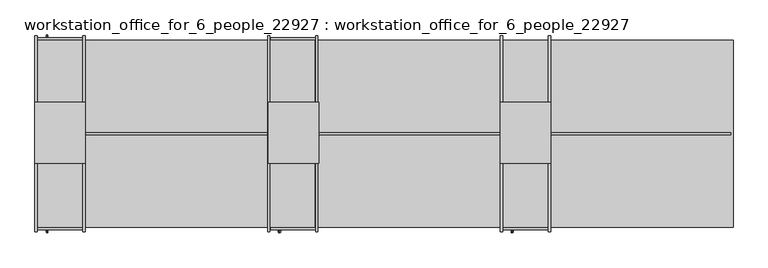
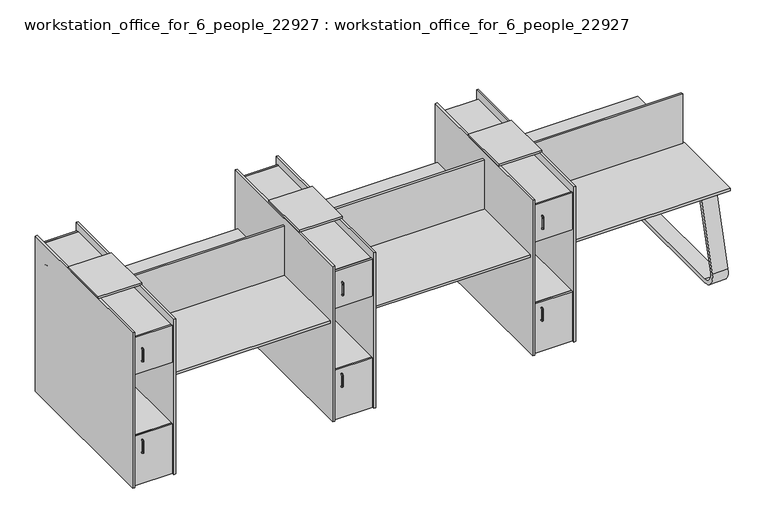
"""IFC4 building model written with IfcOpenShell, lengths in millimetres: proxy geometry, workstation_office_for_6_people_22927 : workstation_office_for_6_people_22927."""

from ifc_helpers import new_model, si_unit, point, frame, frame_2d, origin, origin_with_axes, place, context, project, spatial, polyline, circle_curve, ellipse_curve, trimmed, segment, composite_curve, outline, extrude, source, transform, mapped, element, save
from ifc_brep_helpers import plane_surface, cylinder_surface, revolved_surface, advanced_brep


def workstation_office_for_6_people_22927_workstation_office_for_5136932c(model_context):
    return source(origin(), model_context, "Body", "SolidModel", [
        extrude(outline(polyline([(600.0, 615.0), (600.0, -615.0), (-600.0, -615.0), (-600.0, 615.0), (600.0, 615.0)])), frame((0.0, 0.0, 780.0), z_axis=(0.0, 0.0, 1.0), x_axis=(1.0, 0.0, 0.0)), (0.0, 0.0, 1.0), 20.0),
        extrude(outline(polyline([(2130.0, 615.0), (2130.0, -615.0), (930.0, -615.0), (930.0, 615.0), (2130.0, 615.0)])), frame((0.0, 0.0, 780.0), z_axis=(0.0, 0.0, 1.0), x_axis=(1.0, 0.0, 0.0)), (0.0, 0.0, 1.0), 20.0),
        extrude(outline(polyline([(3660.0, 615.0), (3660.0, -615.0), (2460.0, -615.0), (2460.0, 615.0), (3660.0, 615.0)])), frame((0.0, 0.0, 780.0), z_axis=(0.0, 0.0, 1.0), x_axis=(1.0, 0.0, 0.0)), (0.0, 0.0, 1.0), 20.0),
        extrude(outline(polyline([(600.0, 7.5), (600.0, -7.5), (-600.0, -7.5), (-600.0, 7.5), (600.0, 7.5)])), frame((0.0, 0.0, 400.0), z_axis=(0.0, 0.0, 1.0), x_axis=(1.0, 0.0, 0.0)), (0.0, 0.0, 1.0), 800.0),
        extrude(outline(polyline([(615.0, 645.0), (615.0, -645.0), (600.0, -645.0), (600.0, 645.0), (615.0, 645.0)])), origin_with_axes(), (0.0, 0.0, 1.0), 1256.9637679),
        extrude(outline(polyline([(-615.0, 645.0), (-600.0, 645.0), (-600.0, -645.0), (-615.0, -645.0), (-615.0, 645.0)])), origin_with_axes(), (0.0, 0.0, 1.0), 1256.9637679),
        extrude(outline(polyline([(930.0, 645.0), (930.0, -645.0), (915.0, -645.0), (915.0, 645.0), (930.0, 645.0)])), origin_with_axes(), (0.0, 0.0, 1.0), 1256.9637679),
        extrude(outline(polyline([(-930.0, 645.0), (-915.0, 645.0), (-915.0, -645.0), (-930.0, -645.0), (-930.0, 645.0)])), origin_with_axes(), (0.0, 0.0, 1.0), 1256.9637679),
        extrude(outline(polyline([(2145.0, 645.0), (2145.0, -645.0), (2130.0, -645.0), (2130.0, 645.0), (2145.0, 645.0)])), origin_with_axes(), (0.0, 0.0, 1.0), 1256.9637679),
        extrude(outline(polyline([(2460.0, 645.0), (2460.0, -645.0), (2445.0, -645.0), (2445.0, 645.0), (2460.0, 645.0)])), origin_with_axes(), (0.0, 0.0, 1.0), 1256.9637679),
        extrude(outline(polyline([(-615.0, 615.0), (-615.0, -615.0), (-915.0, -615.0), (-915.0, 615.0), (-615.0, 615.0)])), origin_with_axes(), (0.0, 0.0, 1.0), 400.0),
        extrude(outline(polyline([(615.0, 615.0), (915.0, 615.0), (915.0, -615.0), (615.0, -615.0), (615.0, 615.0)])), origin_with_axes(), (0.0, 0.0, 1.0), 400.0),
        extrude(outline(polyline([(2145.0, 615.0), (2445.0, 615.0), (2445.0, -615.0), (2145.0, -615.0), (2145.0, 615.0)])), origin_with_axes(), (0.0, 0.0, 1.0), 400.0),
        extrude(outline(polyline([(-620.0, 615.0), (-620.0, -615.0), (-920.0, -615.0), (-920.0, 615.0), (-620.0, 615.0)])), frame((0.0, 0.0, 900.0), z_axis=(0.0, 0.0, 1.0), x_axis=(1.0, 0.0, 0.0)), (0.0, 0.0, 1.0), 300.0),
        extrude(outline(polyline([(610.0, 615.0), (910.0, 615.0), (910.0, -615.0), (610.0, -615.0), (610.0, 615.0)])), frame((0.0, 0.0, 900.0), z_axis=(0.0, 0.0, 1.0), x_axis=(1.0, 0.0, 0.0)), (0.0, 0.0, 1.0), 300.0),
        extrude(outline(polyline([(2140.0, 615.0), (2440.0, 615.0), (2440.0, -615.0), (2140.0, -615.0), (2140.0, 615.0)])), frame((0.0, 0.0, 900.0), z_axis=(0.0, 0.0, 1.0), x_axis=(1.0, 0.0, 0.0)), (0.0, 0.0, 1.0), 300.0),
        extrude(outline(polyline([(-620.0, 7.5), (-620.0, -7.5), (-920.0, -7.5), (-920.0, 7.5), (-620.0, 7.5)])), frame((0.0, 0.0, 400.0), z_axis=(0.0, 0.0, 1.0), x_axis=(1.0, 0.0, 0.0)), (0.0, 0.0, 1.0), 500.0),
        extrude(outline(polyline([(610.0, 7.5), (910.0, 7.5), (910.0, -7.5), (610.0, -7.5), (610.0, 7.5)])), frame((0.0, 0.0, 400.0), z_axis=(0.0, 0.0, 1.0), x_axis=(1.0, 0.0, 0.0)), (0.0, 0.0, 1.0), 500.0),
        extrude(outline(polyline([(-620.0, -629.8015658), (-920.0, -629.8015658), (-920.0, -615.0), (-620.0, -615.0), (-620.0, -629.8015658)])), frame((0.0, 0.0, 900.0), z_axis=(0.0, 0.0, 1.0), x_axis=(1.0, 0.0, 0.0)), (0.0, 0.0, 1.0), 300.0),
        extrude(outline(polyline([(-615.0, -629.8015658), (-915.0, -629.8015658), (-915.0, -615.0), (-615.0, -615.0), (-615.0, -629.8015658)])), origin_with_axes(), (0.0, 0.0, 1.0), 400.0),
        extrude(outline(polyline([(920.0, -629.8015658), (620.0, -629.8015658), (620.0, -615.0), (920.0, -615.0), (920.0, -629.8015658)])), frame((0.0, 0.0, 900.0), z_axis=(0.0, 0.0, 1.0), x_axis=(1.0, 0.0, 0.0)), (0.0, 0.0, 1.0), 300.0),
        extrude(outline(polyline([(915.0, -629.8015658), (615.0, -629.8015658), (615.0, -615.0), (915.0, -615.0), (915.0, -629.8015658)])), origin_with_axes(), (0.0, 0.0, 1.0), 400.0),
        extrude(outline(polyline([(2450.0, -629.8015658), (2150.0, -629.8015658), (2150.0, -615.0), (2450.0, -615.0), (2450.0, -629.8015658)])), frame((0.0, 0.0, 900.0), z_axis=(0.0, 0.0, 1.0), x_axis=(1.0, 0.0, 0.0)), (0.0, 0.0, 1.0), 300.0),
        extrude(outline(polyline([(2445.0, -629.8015658), (2145.0, -629.8015658), (2145.0, -615.0), (2445.0, -615.0), (2445.0, -629.8015658)])), origin_with_axes(), (0.0, 0.0, 1.0), 400.0),
        extrude(outline(polyline([(-920.0, 629.8015658), (-620.0, 629.8015658), (-620.0, 615.0), (-920.0, 615.0), (-920.0, 629.8015658)])), frame((0.0, 0.0, 900.0), z_axis=(0.0, 0.0, 1.0), x_axis=(1.0, 0.0, 0.0)), (0.0, 0.0, 1.0), 300.0),
        extrude(outline(polyline([(-915.0, 629.8015658), (-615.0, 629.8015658), (-615.0, 615.0), (-915.0, 615.0), (-915.0, 629.8015658)])), origin_with_axes(), (0.0, 0.0, 1.0), 400.0),
        extrude(outline(polyline([(620.0, 629.8015658), (920.0, 629.8015658), (920.0, 615.0), (620.0, 615.0), (620.0, 629.8015658)])), frame((0.0, 0.0, 900.0), z_axis=(0.0, 0.0, 1.0), x_axis=(1.0, 0.0, 0.0)), (0.0, 0.0, 1.0), 300.0),
        extrude(outline(polyline([(615.0, 629.8015658), (915.0, 629.8015658), (915.0, 615.0), (615.0, 615.0), (615.0, 629.8015658)])), origin_with_axes(), (0.0, 0.0, 1.0), 400.0),
        extrude(outline(polyline([(2130.0, 7.5), (2130.0, -7.5), (930.0, -7.5), (930.0, 7.5), (2130.0, 7.5)])), frame((0.0, 0.0, 400.0), z_axis=(0.0, 0.0, 1.0), x_axis=(1.0, 0.0, 0.0)), (0.0, 0.0, 1.0), 800.0),
        extrude(outline(polyline([(3644.2536992, 7.5), (3644.2536992, -7.5), (2460.0, -7.5), (2460.0, 7.5), (3644.2536992, 7.5)])), frame((0.0, 0.0, 400.0), z_axis=(0.0, 0.0, 1.0), x_axis=(1.0, 0.0, 0.0)), (0.0, 0.0, 1.0), 800.0),
        extrude(outline(composite_curve([segment(polyline([(483.7065392, 0.0), (-483.7065392, 0.0)]), True, "CONTINUOUS"), segment(trimmed(circle_curve(frame_2d((-483.7065392, 100.0)), 100.0), [point((-483.7065392, 0.0))], [point((-580.1112618, 126.5730966))], False, "CARTESIAN"), True, "CONTINUOUS"), segment(polyline([(-580.1112618, 126.5730966), (-420.239467, 706.5730966)]), True, "CONTINUOUS"), segment(trimmed(circle_curve(frame_2d((-323.8347444, 680.0)), 100.0), [point((-420.239467, 706.5730966))], [point((-323.8347444, 780.0))], False, "CARTESIAN"), True, "CONTINUOUS"), segment(polyline([(-323.8347444, 780.0), (323.8347444, 780.0)]), True, "CONTINUOUS"), segment(trimmed(circle_curve(frame_2d((323.8347444, 680.0)), 100.0), [point((323.8347444, 780.0))], [point((420.239467, 706.5730966))], False, "CARTESIAN"), True, "CONTINUOUS"), segment(polyline([(420.239467, 706.5730966), (580.1112618, 126.5730966)]), True, "CONTINUOUS"), segment(trimmed(circle_curve(frame_2d((483.7065392, 100.0)), 100.0), [point((580.1112618, 126.5730966))], [point((483.7065392, 0.0))], False, "CARTESIAN"), True, "CONTINUOUS")], self_intersect=False), holes=[composite_curve([segment(trimmed(circle_curve(frame_2d((-323.8347444, 680.0)), 70.0), [point((-323.8347444, 750.0))], [point((-391.3180502, 698.6011676))], True, "CARTESIAN"), True, "CONTINUOUS"), segment(polyline([(-391.3180502, 698.6011676), (-551.1898451, 118.6011676)]), True, "CONTINUOUS"), segment(trimmed(circle_curve(frame_2d((-483.7065392, 100.0)), 70.0), [point((-551.1898451, 118.6011676))], [point((-483.7065392, 30.0))], True, "CARTESIAN"), True, "CONTINUOUS"), segment(polyline([(-483.7065392, 30.0), (483.7065392, 30.0)]), True, "CONTINUOUS"), segment(trimmed(circle_curve(frame_2d((483.7065392, 100.0)), 70.0), [point((483.7065392, 30.0))], [point((551.1898451, 118.6011676))], True, "CARTESIAN"), True, "CONTINUOUS"), segment(polyline([(551.1898451, 118.6011676), (391.3180502, 698.6011676)]), True, "CONTINUOUS"), segment(trimmed(circle_curve(frame_2d((323.8347444, 680.0)), 70.0), [point((391.3180502, 698.6011676))], [point((323.8347444, 750.0))], True, "CARTESIAN"), True, "CONTINUOUS"), segment(polyline([(323.8347444, 750.0), (-323.8347444, 750.0)]), True, "CONTINUOUS")], self_intersect=False)]), frame((3540.9206772, 0.0, 0.0), z_axis=(1.0, 0.0, 0.0), x_axis=(0.0, 1.0, 0.0)), (0.0, 0.0, 1.0), 119.0793228),
        extrude(outline(polyline([(-930.0, -192.5), (-930.0, 207.5), (-600.0, 207.5), (-600.0, -192.5), (-930.0, -192.5)])), frame((0.0, 0.0, 1256.9637679), z_axis=(0.0, 0.0, 1.0), x_axis=(1.0, 0.0, 0.0)), (0.0, 0.0, 1.0), 16.6578546),
        extrude(outline(polyline([(605.0, -192.5), (605.0, 207.5), (935.0, 207.5), (935.0, -192.5), (605.0, -192.5)])), frame((0.0, 0.0, 1256.9637679), z_axis=(0.0, 0.0, 1.0), x_axis=(1.0, 0.0, 0.0)), (0.0, 0.0, 1.0), 16.6578546),
        extrude(outline(polyline([(2130.0, -192.5), (2130.0, 207.5), (2460.0, 207.5), (2460.0, -192.5), (2130.0, -192.5)])), frame((0.0, 0.0, 1256.9637679), z_axis=(0.0, 0.0, 1.0), x_axis=(1.0, 0.0, 0.0)), (0.0, 0.0, 1.0), 16.6578546),
        advanced_brep(
        [(-850.0, -629.8015658, 1100.0), (-850.0, -629.8015658, 1090.0), (-850.0, -635.0, 1100.0), (-850.0, -635.0, 1090.0), (-850.0, -640.0, 1085.0), (-850.0, -650.0, 1085.0), (-850.0, -650.0, 1005.0), (-850.0, -640.0, 1005.0), (-850.0, -635.0, 1000.0), (-850.0, -635.0, 990.0), (-850.0, -629.8015658, 990.0), (-850.0, -629.8015658, 1000.0)],
        [
            (0, 1, circle_curve(frame((-850.0, -629.8015658, 1095.0), z_axis=(0.0, 1.0, 0.0), x_axis=(0.0, 0.0, -1.0)), 5.0)),
            (1, 0, circle_curve(frame((-850.0, -629.8015658, 1095.0), z_axis=(0.0, 1.0, 0.0), x_axis=(0.0, 0.0, -1.0)), 5.0)),
            (0, 2),
            (2, 3, circle_curve(frame((-850.0, -635.0, 1095.0), z_axis=(0.0, 1.0, 0.0), x_axis=(0.0, 0.0, -1.0)), 5.0)),
            (3, 1),
            (3, 2, circle_curve(frame((-850.0, -635.0, 1095.0), z_axis=(0.0, 1.0, 0.0), x_axis=(0.0, 0.0, -1.0)), 5.0)),
            (4, 3, circle_curve(frame((-850.0, -635.0, 1085.0), z_axis=(-1.0, 0.0, 0.0), x_axis=(0.0, 0.0, 1.0)), 5.0)),
            (2, 5, circle_curve(frame((-850.0, -635.0, 1085.0), z_axis=(1.0, 0.0, 0.0), x_axis=(0.0, 0.0, 1.0)), 15.0)),
            (5, 4, circle_curve(frame((-850.0, -645.0, 1085.0), z_axis=(0.0, 0.0, 1.0), x_axis=(0.0, 1.0, 0.0)), 5.0)),
            (4, 5, circle_curve(frame((-850.0, -645.0, 1085.0), z_axis=(0.0, 0.0, 1.0), x_axis=(0.0, 1.0, 0.0)), 5.0)),
            (5, 6),
            (6, 7, circle_curve(frame((-850.0, -645.0, 1005.0), z_axis=(0.0, 0.0, 1.0), x_axis=(0.0, 1.0, 0.0)), 5.0)),
            (7, 4),
            (7, 6, circle_curve(frame((-850.0, -645.0, 1005.0), z_axis=(0.0, 0.0, 1.0), x_axis=(0.0, 1.0, 0.0)), 5.0)),
            (8, 7, circle_curve(frame((-850.0, -635.0, 1005.0), z_axis=(-1.0, 0.0, 0.0), x_axis=(0.0, -1.0, 0.0)), 5.0)),
            (6, 9, circle_curve(frame((-850.0, -635.0, 1005.0), z_axis=(1.0, 0.0, 0.0), x_axis=(0.0, -1.0, 0.0)), 15.0)),
            (9, 8, circle_curve(frame((-850.0, -635.0, 995.0), z_axis=(0.0, -1.0, 0.0), x_axis=(0.0, 0.0, 1.0)), 5.0)),
            (8, 9, circle_curve(frame((-850.0, -635.0, 995.0), z_axis=(0.0, -1.0, 0.0), x_axis=(0.0, 0.0, 1.0)), 5.0)),
            (10, 11, circle_curve(frame((-850.0, -629.8015658, 995.0), z_axis=(0.0, 1.0, 0.0), x_axis=(0.0, 0.0, 1.0)), 5.0)),
            (11, 10, circle_curve(frame((-850.0, -629.8015658, 995.0), z_axis=(0.0, 1.0, 0.0), x_axis=(0.0, 0.0, 1.0)), 5.0)),
            (9, 10),
            (11, 8),
        ],
        [
            plane_surface(frame((0.0, -629.8015658, 1095.0), z_axis=(0.0, 1.0, 0.0), x_axis=(1.0, 0.0, 0.0))),
            cylinder_surface(frame((-850.0, -629.8015658, 1095.0), z_axis=(0.0, 1.0, 0.0), x_axis=(0.0, 0.0, -1.0)), 5.0),
            revolved_surface(trimmed(ellipse_curve(frame((-850.0, -635.0, 1095.0), z_axis=(0.0, 1.0, 0.0), x_axis=(0.0, 0.0, -1.0)), 5.0, 5.0), [point((-850.0, -635.0, 1100.0))], [point((-850.0, -635.0, 1090.0))], True, "CARTESIAN"), (0.0, -635.0, 1085.0), (1.0, 0.0, 0.0)),
            revolved_surface(trimmed(ellipse_curve(frame((-850.0, -635.0, 1095.0), z_axis=(0.0, 1.0, 0.0), x_axis=(0.0, 0.0, -1.0)), 5.0, 5.0), [point((-850.0, -635.0, 1090.0))], [point((-850.0, -635.0, 1100.0))], True, "CARTESIAN"), (0.0, -635.0, 1085.0), (1.0, 0.0, 0.0)),
            cylinder_surface(frame((-850.0, -645.0, 1085.0), z_axis=(0.0, 0.0, 1.0), x_axis=(0.0, 1.0, 0.0)), 5.0),
            revolved_surface(trimmed(ellipse_curve(frame((-850.0, -645.0, 1005.0), z_axis=(0.0, 0.0, 1.0), x_axis=(0.0, 1.0, 0.0)), 5.0, 5.0), [point((-850.0, -650.0, 1005.0))], [point((-850.0, -640.0, 1005.0))], True, "CARTESIAN"), (0.0, -635.0, 1005.0), (1.0, 0.0, 0.0)),
            revolved_surface(trimmed(ellipse_curve(frame((-850.0, -645.0, 1005.0), z_axis=(0.0, 0.0, 1.0), x_axis=(0.0, 1.0, 0.0)), 5.0, 5.0), [point((-850.0, -640.0, 1005.0))], [point((-850.0, -650.0, 1005.0))], True, "CARTESIAN"), (0.0, -635.0, 1005.0), (1.0, 0.0, 0.0)),
            plane_surface(frame((0.0, -629.8015658, 995.0), z_axis=(0.0, 1.0, 0.0), x_axis=(1.0, 0.0, 0.0))),
            cylinder_surface(frame((-850.0, -635.0, 995.0), z_axis=(0.0, -1.0, 0.0), x_axis=(0.0, 0.0, 1.0)), 5.0),
        ],
        [
            (0, [[1, 2]]),
            (1, [[-1, 3, 4, 5]]),
            (1, [[-2, -5, 6, -3]]),
            (2, [[7, -4, 8, 9]]),
            (3, [[-8, -6, -7, 10]]),
            (4, [[-9, 11, 12, 13]]),
            (4, [[-10, -13, 14, -11]]),
            (5, [[15, -12, 16, 17]]),
            (6, [[-16, -14, -15, 18]]),
            (7, [[19, 20]]),
            (8, [[-17, 21, -20, 22]]),
            (8, [[-18, -22, -19, -21]]),
        ],
    ),
        advanced_brep(
        [(-850.0, -629.8015658, 360.0), (-850.0, -629.8015658, 350.0), (-850.0, -635.0, 360.0), (-850.0, -635.0, 350.0), (-850.0, -640.0, 345.0), (-850.0, -650.0, 345.0), (-850.0, -650.0, 265.0), (-850.0, -640.0, 265.0), (-850.0, -635.0, 260.0), (-850.0, -635.0, 250.0), (-850.0, -629.8015658, 250.0), (-850.0, -629.8015658, 260.0)],
        [
            (0, 1, circle_curve(frame((-850.0, -629.8015658, 355.0), z_axis=(0.0, 1.0, 0.0), x_axis=(0.0, 0.0, -1.0)), 5.0)),
            (1, 0, circle_curve(frame((-850.0, -629.8015658, 355.0), z_axis=(0.0, 1.0, 0.0), x_axis=(0.0, 0.0, -1.0)), 5.0)),
            (0, 2),
            (2, 3, circle_curve(frame((-850.0, -635.0, 355.0), z_axis=(0.0, 1.0, 0.0), x_axis=(0.0, 0.0, -1.0)), 5.0)),
            (3, 1),
            (3, 2, circle_curve(frame((-850.0, -635.0, 355.0), z_axis=(0.0, 1.0, 0.0), x_axis=(0.0, 0.0, -1.0)), 5.0)),
            (4, 3, circle_curve(frame((-850.0, -635.0, 345.0), z_axis=(-1.0, 0.0, 0.0), x_axis=(0.0, 0.0, 1.0)), 5.0)),
            (2, 5, circle_curve(frame((-850.0, -635.0, 345.0), z_axis=(1.0, 0.0, 0.0), x_axis=(0.0, 0.0, 1.0)), 15.0)),
            (5, 4, circle_curve(frame((-850.0, -645.0, 345.0), z_axis=(0.0, 0.0, 1.0), x_axis=(0.0, 1.0, 0.0)), 5.0)),
            (4, 5, circle_curve(frame((-850.0, -645.0, 345.0), z_axis=(0.0, 0.0, 1.0), x_axis=(0.0, 1.0, 0.0)), 5.0)),
            (5, 6),
            (6, 7, circle_curve(frame((-850.0, -645.0, 265.0), z_axis=(0.0, 0.0, 1.0), x_axis=(0.0, 1.0, 0.0)), 5.0)),
            (7, 4),
            (7, 6, circle_curve(frame((-850.0, -645.0, 265.0), z_axis=(0.0, 0.0, 1.0), x_axis=(0.0, 1.0, 0.0)), 5.0)),
            (8, 7, circle_curve(frame((-850.0, -635.0, 265.0), z_axis=(-1.0, 0.0, 0.0), x_axis=(0.0, -1.0, 0.0)), 5.0)),
            (6, 9, circle_curve(frame((-850.0, -635.0, 265.0), z_axis=(1.0, 0.0, 0.0), x_axis=(0.0, -1.0, 0.0)), 15.0)),
            (9, 8, circle_curve(frame((-850.0, -635.0, 255.0), z_axis=(0.0, -1.0, 0.0), x_axis=(0.0, 0.0, 1.0)), 5.0)),
            (8, 9, circle_curve(frame((-850.0, -635.0, 255.0), z_axis=(0.0, -1.0, 0.0), x_axis=(0.0, 0.0, 1.0)), 5.0)),
            (10, 11, circle_curve(frame((-850.0, -629.8015658, 255.0), z_axis=(0.0, 1.0, 0.0), x_axis=(0.0, 0.0, 1.0)), 5.0)),
            (11, 10, circle_curve(frame((-850.0, -629.8015658, 255.0), z_axis=(0.0, 1.0, 0.0), x_axis=(0.0, 0.0, 1.0)), 5.0)),
            (9, 10),
            (11, 8),
        ],
        [
            plane_surface(frame((0.0, -629.8015658, 355.0), z_axis=(0.0, 1.0, 0.0), x_axis=(1.0, 0.0, 0.0))),
            cylinder_surface(frame((-850.0, -629.8015658, 355.0), z_axis=(0.0, 1.0, 0.0), x_axis=(0.0, 0.0, -1.0)), 5.0),
            revolved_surface(trimmed(ellipse_curve(frame((-850.0, -635.0, 355.0), z_axis=(0.0, 1.0, 0.0), x_axis=(0.0, 0.0, -1.0)), 5.0, 5.0), [point((-850.0, -635.0, 360.0))], [point((-850.0, -635.0, 350.0))], True, "CARTESIAN"), (0.0, -635.0, 345.0), (1.0, 0.0, 0.0)),
            revolved_surface(trimmed(ellipse_curve(frame((-850.0, -635.0, 355.0), z_axis=(0.0, 1.0, 0.0), x_axis=(0.0, 0.0, -1.0)), 5.0, 5.0), [point((-850.0, -635.0, 350.0))], [point((-850.0, -635.0, 360.0))], True, "CARTESIAN"), (0.0, -635.0, 345.0), (1.0, 0.0, 0.0)),
            cylinder_surface(frame((-850.0, -645.0, 345.0), z_axis=(0.0, 0.0, 1.0), x_axis=(0.0, 1.0, 0.0)), 5.0),
            revolved_surface(trimmed(ellipse_curve(frame((-850.0, -645.0, 265.0), z_axis=(0.0, 0.0, 1.0), x_axis=(0.0, 1.0, 0.0)), 5.0, 5.0), [point((-850.0, -650.0, 265.0))], [point((-850.0, -640.0, 265.0))], True, "CARTESIAN"), (0.0, -635.0, 265.0), (1.0, 0.0, 0.0)),
            revolved_surface(trimmed(ellipse_curve(frame((-850.0, -645.0, 265.0), z_axis=(0.0, 0.0, 1.0), x_axis=(0.0, 1.0, 0.0)), 5.0, 5.0), [point((-850.0, -640.0, 265.0))], [point((-850.0, -650.0, 265.0))], True, "CARTESIAN"), (0.0, -635.0, 265.0), (1.0, 0.0, 0.0)),
            plane_surface(frame((0.0, -629.8015658, 255.0), z_axis=(0.0, 1.0, 0.0), x_axis=(1.0, 0.0, 0.0))),
            cylinder_surface(frame((-850.0, -635.0, 255.0), z_axis=(0.0, -1.0, 0.0), x_axis=(0.0, 0.0, 1.0)), 5.0),
        ],
        [
            (0, [[1, 2]]),
            (1, [[-1, 3, 4, 5]]),
            (1, [[-2, -5, 6, -3]]),
            (2, [[7, -4, 8, 9]]),
            (3, [[-8, -6, -7, 10]]),
            (4, [[-9, 11, 12, 13]]),
            (4, [[-10, -13, 14, -11]]),
            (5, [[15, -12, 16, 17]]),
            (6, [[-16, -14, -15, 18]]),
            (7, [[19, 20]]),
            (8, [[-17, 21, -20, 22]]),
            (8, [[-18, -22, -19, -21]]),
        ],
    ),
        advanced_brep(
        [(680.0, -629.8015658, 1100.0), (680.0, -629.8015658, 1090.0), (680.0, -635.0, 1100.0), (680.0, -635.0, 1090.0), (680.0, -640.0, 1085.0), (680.0, -650.0, 1085.0), (680.0, -650.0, 1005.0), (680.0, -640.0, 1005.0), (680.0, -635.0, 1000.0), (680.0, -635.0, 990.0), (680.0, -629.8015658, 990.0), (680.0, -629.8015658, 1000.0)],
        [
            (0, 1, circle_curve(frame((680.0, -629.8015658, 1095.0), z_axis=(0.0, 1.0, 0.0), x_axis=(0.0, 0.0, -1.0)), 5.0)),
            (1, 0, circle_curve(frame((680.0, -629.8015658, 1095.0), z_axis=(0.0, 1.0, 0.0), x_axis=(0.0, 0.0, -1.0)), 5.0)),
            (0, 2),
            (2, 3, circle_curve(frame((680.0, -635.0, 1095.0), z_axis=(0.0, 1.0, 0.0), x_axis=(0.0, 0.0, -1.0)), 5.0)),
            (3, 1),
            (3, 2, circle_curve(frame((680.0, -635.0, 1095.0), z_axis=(0.0, 1.0, 0.0), x_axis=(0.0, 0.0, -1.0)), 5.0)),
            (4, 3, circle_curve(frame((680.0, -635.0, 1085.0), z_axis=(-1.0, 0.0, 0.0), x_axis=(0.0, 0.0, 1.0)), 5.0)),
            (2, 5, circle_curve(frame((680.0, -635.0, 1085.0), z_axis=(1.0, 0.0, 0.0), x_axis=(0.0, 0.0, 1.0)), 15.0)),
            (5, 4, circle_curve(frame((680.0, -645.0, 1085.0), z_axis=(0.0, 0.0, 1.0), x_axis=(0.0, 1.0, 0.0)), 5.0)),
            (4, 5, circle_curve(frame((680.0, -645.0, 1085.0), z_axis=(0.0, 0.0, 1.0), x_axis=(0.0, 1.0, 0.0)), 5.0)),
            (5, 6),
            (6, 7, circle_curve(frame((680.0, -645.0, 1005.0), z_axis=(0.0, 0.0, 1.0), x_axis=(0.0, 1.0, 0.0)), 5.0)),
            (7, 4),
            (7, 6, circle_curve(frame((680.0, -645.0, 1005.0), z_axis=(0.0, 0.0, 1.0), x_axis=(0.0, 1.0, 0.0)), 5.0)),
            (8, 7, circle_curve(frame((680.0, -635.0, 1005.0), z_axis=(-1.0, 0.0, 0.0), x_axis=(0.0, -1.0, 0.0)), 5.0)),
            (6, 9, circle_curve(frame((680.0, -635.0, 1005.0), z_axis=(1.0, 0.0, 0.0), x_axis=(0.0, -1.0, 0.0)), 15.0)),
            (9, 8, circle_curve(frame((680.0, -635.0, 995.0), z_axis=(0.0, -1.0, 0.0), x_axis=(0.0, 0.0, 1.0)), 5.0)),
            (8, 9, circle_curve(frame((680.0, -635.0, 995.0), z_axis=(0.0, -1.0, 0.0), x_axis=(0.0, 0.0, 1.0)), 5.0)),
            (10, 11, circle_curve(frame((680.0, -629.8015658, 995.0), z_axis=(0.0, 1.0, 0.0), x_axis=(0.0, 0.0, 1.0)), 5.0)),
            (11, 10, circle_curve(frame((680.0, -629.8015658, 995.0), z_axis=(0.0, 1.0, 0.0), x_axis=(0.0, 0.0, 1.0)), 5.0)),
            (9, 10),
            (11, 8),
        ],
        [
            plane_surface(frame((1530.0, -629.8015658, 1095.0), z_axis=(0.0, 1.0, 0.0), x_axis=(1.0, 0.0, 0.0))),
            cylinder_surface(frame((680.0, -629.8015658, 1095.0), z_axis=(0.0, 1.0, 0.0), x_axis=(0.0, 0.0, -1.0)), 5.0),
            revolved_surface(trimmed(ellipse_curve(frame((680.0, -635.0, 1095.0), z_axis=(0.0, 1.0, 0.0), x_axis=(0.0, 0.0, -1.0)), 5.0, 5.0), [point((680.0, -635.0, 1100.0))], [point((680.0, -635.0, 1090.0))], True, "CARTESIAN"), (1530.0, -635.0, 1085.0), (1.0, 0.0, 0.0)),
            revolved_surface(trimmed(ellipse_curve(frame((680.0, -635.0, 1095.0), z_axis=(0.0, 1.0, 0.0), x_axis=(0.0, 0.0, -1.0)), 5.0, 5.0), [point((680.0, -635.0, 1090.0))], [point((680.0, -635.0, 1100.0))], True, "CARTESIAN"), (1530.0, -635.0, 1085.0), (1.0, 0.0, 0.0)),
            cylinder_surface(frame((680.0, -645.0, 1085.0), z_axis=(0.0, 0.0, 1.0), x_axis=(0.0, 1.0, 0.0)), 5.0),
            revolved_surface(trimmed(ellipse_curve(frame((680.0, -645.0, 1005.0), z_axis=(0.0, 0.0, 1.0), x_axis=(0.0, 1.0, 0.0)), 5.0, 5.0), [point((680.0, -650.0, 1005.0))], [point((680.0, -640.0, 1005.0))], True, "CARTESIAN"), (1530.0, -635.0, 1005.0), (1.0, 0.0, 0.0)),
            revolved_surface(trimmed(ellipse_curve(frame((680.0, -645.0, 1005.0), z_axis=(0.0, 0.0, 1.0), x_axis=(0.0, 1.0, 0.0)), 5.0, 5.0), [point((680.0, -640.0, 1005.0))], [point((680.0, -650.0, 1005.0))], True, "CARTESIAN"), (1530.0, -635.0, 1005.0), (1.0, 0.0, 0.0)),
            plane_surface(frame((1530.0, -629.8015658, 995.0), z_axis=(0.0, 1.0, 0.0), x_axis=(1.0, 0.0, 0.0))),
            cylinder_surface(frame((680.0, -635.0, 995.0), z_axis=(0.0, -1.0, 0.0), x_axis=(0.0, 0.0, 1.0)), 5.0),
        ],
        [
            (0, [[1, 2]]),
            (1, [[-1, 3, 4, 5]]),
            (1, [[-2, -5, 6, -3]]),
            (2, [[7, -4, 8, 9]]),
            (3, [[-8, -6, -7, 10]]),
            (4, [[-9, 11, 12, 13]]),
            (4, [[-10, -13, 14, -11]]),
            (5, [[15, -12, 16, 17]]),
            (6, [[-16, -14, -15, 18]]),
            (7, [[19, 20]]),
            (8, [[-17, 21, -20, 22]]),
            (8, [[-18, -22, -19, -21]]),
        ],
    ),
        advanced_brep(
        [(675.0, -629.8015658, 360.0), (675.0, -629.8015658, 350.0), (675.0, -635.0, 360.0), (675.0, -635.0, 350.0), (675.0, -640.0, 345.0), (675.0, -650.0, 345.0), (675.0, -650.0, 265.0), (675.0, -640.0, 265.0), (675.0, -635.0, 260.0), (675.0, -635.0, 250.0), (675.0, -629.8015658, 250.0), (675.0, -629.8015658, 260.0)],
        [
            (0, 1, circle_curve(frame((675.0, -629.8015658, 355.0), z_axis=(0.0, 1.0, 0.0), x_axis=(0.0, 0.0, -1.0)), 5.0)),
            (1, 0, circle_curve(frame((675.0, -629.8015658, 355.0), z_axis=(0.0, 1.0, 0.0), x_axis=(0.0, 0.0, -1.0)), 5.0)),
            (0, 2),
            (2, 3, circle_curve(frame((675.0, -635.0, 355.0), z_axis=(0.0, 1.0, 0.0), x_axis=(0.0, 0.0, -1.0)), 5.0)),
            (3, 1),
            (3, 2, circle_curve(frame((675.0, -635.0, 355.0), z_axis=(0.0, 1.0, 0.0), x_axis=(0.0, 0.0, -1.0)), 5.0)),
            (4, 3, circle_curve(frame((675.0, -635.0, 345.0), z_axis=(-1.0, 0.0, 0.0), x_axis=(0.0, 0.0, 1.0)), 5.0)),
            (2, 5, circle_curve(frame((675.0, -635.0, 345.0), z_axis=(1.0, 0.0, 0.0), x_axis=(0.0, 0.0, 1.0)), 15.0)),
            (5, 4, circle_curve(frame((675.0, -645.0, 345.0), z_axis=(0.0, 0.0, 1.0), x_axis=(0.0, 1.0, 0.0)), 5.0)),
            (4, 5, circle_curve(frame((675.0, -645.0, 345.0), z_axis=(0.0, 0.0, 1.0), x_axis=(0.0, 1.0, 0.0)), 5.0)),
            (5, 6),
            (6, 7, circle_curve(frame((675.0, -645.0, 265.0), z_axis=(0.0, 0.0, 1.0), x_axis=(0.0, 1.0, 0.0)), 5.0)),
            (7, 4),
            (7, 6, circle_curve(frame((675.0, -645.0, 265.0), z_axis=(0.0, 0.0, 1.0), x_axis=(0.0, 1.0, 0.0)), 5.0)),
            (8, 7, circle_curve(frame((675.0, -635.0, 265.0), z_axis=(-1.0, 0.0, 0.0), x_axis=(0.0, -1.0, 0.0)), 5.0)),
            (6, 9, circle_curve(frame((675.0, -635.0, 265.0), z_axis=(1.0, 0.0, 0.0), x_axis=(0.0, -1.0, 0.0)), 15.0)),
            (9, 8, circle_curve(frame((675.0, -635.0, 255.0), z_axis=(0.0, -1.0, 0.0), x_axis=(0.0, 0.0, 1.0)), 5.0)),
            (8, 9, circle_curve(frame((675.0, -635.0, 255.0), z_axis=(0.0, -1.0, 0.0), x_axis=(0.0, 0.0, 1.0)), 5.0)),
            (10, 11, circle_curve(frame((675.0, -629.8015658, 255.0), z_axis=(0.0, 1.0, 0.0), x_axis=(0.0, 0.0, 1.0)), 5.0)),
            (11, 10, circle_curve(frame((675.0, -629.8015658, 255.0), z_axis=(0.0, 1.0, 0.0), x_axis=(0.0, 0.0, 1.0)), 5.0)),
            (9, 10),
            (11, 8),
        ],
        [
            plane_surface(frame((675.0, -629.8015658, 355.0), z_axis=(0.0, 1.0, 0.0), x_axis=(1.0, 0.0, 0.0))),
            cylinder_surface(frame((675.0, -629.8015658, 355.0), z_axis=(0.0, 1.0, 0.0), x_axis=(0.0, 0.0, -1.0)), 5.0),
            revolved_surface(trimmed(ellipse_curve(frame((675.0, -635.0, 355.0), z_axis=(0.0, 1.0, 0.0), x_axis=(0.0, 0.0, -1.0)), 5.0, 5.0), [point((675.0, -635.0, 360.0))], [point((675.0, -635.0, 350.0))], True, "CARTESIAN"), (675.0, -635.0, 345.0), (1.0, 0.0, 0.0)),
            revolved_surface(trimmed(ellipse_curve(frame((675.0, -635.0, 355.0), z_axis=(0.0, 1.0, 0.0), x_axis=(0.0, 0.0, -1.0)), 5.0, 5.0), [point((675.0, -635.0, 350.0))], [point((675.0, -635.0, 360.0))], True, "CARTESIAN"), (675.0, -635.0, 345.0), (1.0, 0.0, 0.0)),
            cylinder_surface(frame((675.0, -645.0, 345.0), z_axis=(0.0, 0.0, 1.0), x_axis=(0.0, 1.0, 0.0)), 5.0),
            revolved_surface(trimmed(ellipse_curve(frame((675.0, -645.0, 265.0), z_axis=(0.0, 0.0, 1.0), x_axis=(0.0, 1.0, 0.0)), 5.0, 5.0), [point((675.0, -650.0, 265.0))], [point((675.0, -640.0, 265.0))], True, "CARTESIAN"), (675.0, -635.0, 265.0), (1.0, 0.0, 0.0)),
            revolved_surface(trimmed(ellipse_curve(frame((675.0, -645.0, 265.0), z_axis=(0.0, 0.0, 1.0), x_axis=(0.0, 1.0, 0.0)), 5.0, 5.0), [point((675.0, -640.0, 265.0))], [point((675.0, -650.0, 265.0))], True, "CARTESIAN"), (675.0, -635.0, 265.0), (1.0, 0.0, 0.0)),
            plane_surface(frame((675.0, -629.8015658, 255.0), z_axis=(0.0, 1.0, 0.0), x_axis=(1.0, 0.0, 0.0))),
            cylinder_surface(frame((675.0, -635.0, 255.0), z_axis=(0.0, -1.0, 0.0), x_axis=(0.0, 0.0, 1.0)), 5.0),
        ],
        [
            (0, [[1, 2]]),
            (1, [[-1, 3, 4, 5]]),
            (1, [[-2, -5, 6, -3]]),
            (2, [[7, -4, 8, 9]]),
            (3, [[-8, -6, -7, 10]]),
            (4, [[-9, 11, 12, 13]]),
            (4, [[-10, -13, 14, -11]]),
            (5, [[15, -12, 16, 17]]),
            (6, [[-16, -14, -15, 18]]),
            (7, [[19, 20]]),
            (8, [[-17, 21, -20, 22]]),
            (8, [[-18, -22, -19, -21]]),
        ],
    ),
        advanced_brep(
        [(2210.0, -629.8015658, 1100.0), (2210.0, -629.8015658, 1090.0), (2210.0, -635.0, 1100.0), (2210.0, -635.0, 1090.0), (2210.0, -640.0, 1085.0), (2210.0, -650.0, 1085.0), (2210.0, -650.0, 1005.0), (2210.0, -640.0, 1005.0), (2210.0, -635.0, 1000.0), (2210.0, -635.0, 990.0), (2210.0, -629.8015658, 990.0), (2210.0, -629.8015658, 1000.0)],
        [
            (0, 1, circle_curve(frame((2210.0, -629.8015658, 1095.0), z_axis=(0.0, 1.0, 0.0), x_axis=(0.0, 0.0, -1.0)), 5.0)),
            (1, 0, circle_curve(frame((2210.0, -629.8015658, 1095.0), z_axis=(0.0, 1.0, 0.0), x_axis=(0.0, 0.0, -1.0)), 5.0)),
            (0, 2),
            (2, 3, circle_curve(frame((2210.0, -635.0, 1095.0), z_axis=(0.0, 1.0, 0.0), x_axis=(0.0, 0.0, -1.0)), 5.0)),
            (3, 1),
            (3, 2, circle_curve(frame((2210.0, -635.0, 1095.0), z_axis=(0.0, 1.0, 0.0), x_axis=(0.0, 0.0, -1.0)), 5.0)),
            (4, 3, circle_curve(frame((2210.0, -635.0, 1085.0), z_axis=(-1.0, 0.0, 0.0), x_axis=(0.0, 0.0, 1.0)), 5.0)),
            (2, 5, circle_curve(frame((2210.0, -635.0, 1085.0), z_axis=(1.0, 0.0, 0.0), x_axis=(0.0, 0.0, 1.0)), 15.0)),
            (5, 4, circle_curve(frame((2210.0, -645.0, 1085.0), z_axis=(0.0, 0.0, 1.0), x_axis=(0.0, 1.0, 0.0)), 5.0)),
            (4, 5, circle_curve(frame((2210.0, -645.0, 1085.0), z_axis=(0.0, 0.0, 1.0), x_axis=(0.0, 1.0, 0.0)), 5.0)),
            (5, 6),
            (6, 7, circle_curve(frame((2210.0, -645.0, 1005.0), z_axis=(0.0, 0.0, 1.0), x_axis=(0.0, 1.0, 0.0)), 5.0)),
            (7, 4),
            (7, 6, circle_curve(frame((2210.0, -645.0, 1005.0), z_axis=(0.0, 0.0, 1.0), x_axis=(0.0, 1.0, 0.0)), 5.0)),
            (8, 7, circle_curve(frame((2210.0, -635.0, 1005.0), z_axis=(-1.0, 0.0, 0.0), x_axis=(0.0, -1.0, 0.0)), 5.0)),
            (6, 9, circle_curve(frame((2210.0, -635.0, 1005.0), z_axis=(1.0, 0.0, 0.0), x_axis=(0.0, -1.0, 0.0)), 15.0)),
            (9, 8, circle_curve(frame((2210.0, -635.0, 995.0), z_axis=(0.0, -1.0, 0.0), x_axis=(0.0, 0.0, 1.0)), 5.0)),
            (8, 9, circle_curve(frame((2210.0, -635.0, 995.0), z_axis=(0.0, -1.0, 0.0), x_axis=(0.0, 0.0, 1.0)), 5.0)),
            (10, 11, circle_curve(frame((2210.0, -629.8015658, 995.0), z_axis=(0.0, 1.0, 0.0), x_axis=(0.0, 0.0, 1.0)), 5.0)),
            (11, 10, circle_curve(frame((2210.0, -629.8015658, 995.0), z_axis=(0.0, 1.0, 0.0), x_axis=(0.0, 0.0, 1.0)), 5.0)),
            (9, 10),
            (11, 8),
        ],
        [
            plane_surface(frame((3060.0, -629.8015658, 1095.0), z_axis=(0.0, 1.0, 0.0), x_axis=(1.0, 0.0, 0.0))),
            cylinder_surface(frame((2210.0, -629.8015658, 1095.0), z_axis=(0.0, 1.0, 0.0), x_axis=(0.0, 0.0, -1.0)), 5.0),
            revolved_surface(trimmed(ellipse_curve(frame((2210.0, -635.0, 1095.0), z_axis=(0.0, 1.0, 0.0), x_axis=(0.0, 0.0, -1.0)), 5.0, 5.0), [point((2210.0, -635.0, 1100.0))], [point((2210.0, -635.0, 1090.0))], True, "CARTESIAN"), (3060.0, -635.0, 1085.0), (1.0, 0.0, 0.0)),
            revolved_surface(trimmed(ellipse_curve(frame((2210.0, -635.0, 1095.0), z_axis=(0.0, 1.0, 0.0), x_axis=(0.0, 0.0, -1.0)), 5.0, 5.0), [point((2210.0, -635.0, 1090.0))], [point((2210.0, -635.0, 1100.0))], True, "CARTESIAN"), (3060.0, -635.0, 1085.0), (1.0, 0.0, 0.0)),
            cylinder_surface(frame((2210.0, -645.0, 1085.0), z_axis=(0.0, 0.0, 1.0), x_axis=(0.0, 1.0, 0.0)), 5.0),
            revolved_surface(trimmed(ellipse_curve(frame((2210.0, -645.0, 1005.0), z_axis=(0.0, 0.0, 1.0), x_axis=(0.0, 1.0, 0.0)), 5.0, 5.0), [point((2210.0, -650.0, 1005.0))], [point((2210.0, -640.0, 1005.0))], True, "CARTESIAN"), (3060.0, -635.0, 1005.0), (1.0, 0.0, 0.0)),
            revolved_surface(trimmed(ellipse_curve(frame((2210.0, -645.0, 1005.0), z_axis=(0.0, 0.0, 1.0), x_axis=(0.0, 1.0, 0.0)), 5.0, 5.0), [point((2210.0, -640.0, 1005.0))], [point((2210.0, -650.0, 1005.0))], True, "CARTESIAN"), (3060.0, -635.0, 1005.0), (1.0, 0.0, 0.0)),
            plane_surface(frame((3060.0, -629.8015658, 995.0), z_axis=(0.0, 1.0, 0.0), x_axis=(1.0, 0.0, 0.0))),
            cylinder_surface(frame((2210.0, -635.0, 995.0), z_axis=(0.0, -1.0, 0.0), x_axis=(0.0, 0.0, 1.0)), 5.0),
        ],
        [
            (0, [[1, 2]]),
            (1, [[-1, 3, 4, 5]]),
            (1, [[-2, -5, 6, -3]]),
            (2, [[7, -4, 8, 9]]),
            (3, [[-8, -6, -7, 10]]),
            (4, [[-9, 11, 12, 13]]),
            (4, [[-10, -13, 14, -11]]),
            (5, [[15, -12, 16, 17]]),
            (6, [[-16, -14, -15, 18]]),
            (7, [[19, 20]]),
            (8, [[-17, 21, -20, 22]]),
            (8, [[-18, -22, -19, -21]]),
        ],
    ),
        advanced_brep(
        [(2205.0, -629.8015658, 360.0), (2205.0, -629.8015658, 350.0), (2205.0, -635.0, 360.0), (2205.0, -635.0, 350.0), (2205.0, -640.0, 345.0), (2205.0, -650.0, 345.0), (2205.0, -650.0, 265.0), (2205.0, -640.0, 265.0), (2205.0, -635.0, 260.0), (2205.0, -635.0, 250.0), (2205.0, -629.8015658, 250.0), (2205.0, -629.8015658, 260.0)],
        [
            (0, 1, circle_curve(frame((2205.0, -629.8015658, 355.0), z_axis=(0.0, 1.0, 0.0), x_axis=(0.0, 0.0, -1.0)), 5.0)),
            (1, 0, circle_curve(frame((2205.0, -629.8015658, 355.0), z_axis=(0.0, 1.0, 0.0), x_axis=(0.0, 0.0, -1.0)), 5.0)),
            (0, 2),
            (2, 3, circle_curve(frame((2205.0, -635.0, 355.0), z_axis=(0.0, 1.0, 0.0), x_axis=(0.0, 0.0, -1.0)), 5.0)),
            (3, 1),
            (3, 2, circle_curve(frame((2205.0, -635.0, 355.0), z_axis=(0.0, 1.0, 0.0), x_axis=(0.0, 0.0, -1.0)), 5.0)),
            (4, 3, circle_curve(frame((2205.0, -635.0, 345.0), z_axis=(-1.0, 0.0, 0.0), x_axis=(0.0, 0.0, 1.0)), 5.0)),
            (2, 5, circle_curve(frame((2205.0, -635.0, 345.0), z_axis=(1.0, 0.0, 0.0), x_axis=(0.0, 0.0, 1.0)), 15.0)),
            (5, 4, circle_curve(frame((2205.0, -645.0, 345.0), z_axis=(0.0, 0.0, 1.0), x_axis=(0.0, 1.0, 0.0)), 5.0)),
            (4, 5, circle_curve(frame((2205.0, -645.0, 345.0), z_axis=(0.0, 0.0, 1.0), x_axis=(0.0, 1.0, 0.0)), 5.0)),
            (5, 6),
            (6, 7, circle_curve(frame((2205.0, -645.0, 265.0), z_axis=(0.0, 0.0, 1.0), x_axis=(0.0, 1.0, 0.0)), 5.0)),
            (7, 4),
            (7, 6, circle_curve(frame((2205.0, -645.0, 265.0), z_axis=(0.0, 0.0, 1.0), x_axis=(0.0, 1.0, 0.0)), 5.0)),
            (8, 7, circle_curve(frame((2205.0, -635.0, 265.0), z_axis=(-1.0, 0.0, 0.0), x_axis=(0.0, -1.0, 0.0)), 5.0)),
            (6, 9, circle_curve(frame((2205.0, -635.0, 265.0), z_axis=(1.0, 0.0, 0.0), x_axis=(0.0, -1.0, 0.0)), 15.0)),
            (9, 8, circle_curve(frame((2205.0, -635.0, 255.0), z_axis=(0.0, -1.0, 0.0), x_axis=(0.0, 0.0, 1.0)), 5.0)),
            (8, 9, circle_curve(frame((2205.0, -635.0, 255.0), z_axis=(0.0, -1.0, 0.0), x_axis=(0.0, 0.0, 1.0)), 5.0)),
            (10, 11, circle_curve(frame((2205.0, -629.8015658, 255.0), z_axis=(0.0, 1.0, 0.0), x_axis=(0.0, 0.0, 1.0)), 5.0)),
            (11, 10, circle_curve(frame((2205.0, -629.8015658, 255.0), z_axis=(0.0, 1.0, 0.0), x_axis=(0.0, 0.0, 1.0)), 5.0)),
            (9, 10),
            (11, 8),
        ],
        [
            plane_surface(frame((2205.0, -629.8015658, 355.0), z_axis=(0.0, 1.0, 0.0), x_axis=(1.0, 0.0, 0.0))),
            cylinder_surface(frame((2205.0, -629.8015658, 355.0), z_axis=(0.0, 1.0, 0.0), x_axis=(0.0, 0.0, -1.0)), 5.0),
            revolved_surface(trimmed(ellipse_curve(frame((2205.0, -635.0, 355.0), z_axis=(0.0, 1.0, 0.0), x_axis=(0.0, 0.0, -1.0)), 5.0, 5.0), [point((2205.0, -635.0, 360.0))], [point((2205.0, -635.0, 350.0))], True, "CARTESIAN"), (2205.0, -635.0, 345.0), (1.0, 0.0, 0.0)),
            revolved_surface(trimmed(ellipse_curve(frame((2205.0, -635.0, 355.0), z_axis=(0.0, 1.0, 0.0), x_axis=(0.0, 0.0, -1.0)), 5.0, 5.0), [point((2205.0, -635.0, 350.0))], [point((2205.0, -635.0, 360.0))], True, "CARTESIAN"), (2205.0, -635.0, 345.0), (1.0, 0.0, 0.0)),
            cylinder_surface(frame((2205.0, -645.0, 345.0), z_axis=(0.0, 0.0, 1.0), x_axis=(0.0, 1.0, 0.0)), 5.0),
            revolved_surface(trimmed(ellipse_curve(frame((2205.0, -645.0, 265.0), z_axis=(0.0, 0.0, 1.0), x_axis=(0.0, 1.0, 0.0)), 5.0, 5.0), [point((2205.0, -650.0, 265.0))], [point((2205.0, -640.0, 265.0))], True, "CARTESIAN"), (2205.0, -635.0, 265.0), (1.0, 0.0, 0.0)),
            revolved_surface(trimmed(ellipse_curve(frame((2205.0, -645.0, 265.0), z_axis=(0.0, 0.0, 1.0), x_axis=(0.0, 1.0, 0.0)), 5.0, 5.0), [point((2205.0, -640.0, 265.0))], [point((2205.0, -650.0, 265.0))], True, "CARTESIAN"), (2205.0, -635.0, 265.0), (1.0, 0.0, 0.0)),
            plane_surface(frame((2205.0, -629.8015658, 255.0), z_axis=(0.0, 1.0, 0.0), x_axis=(1.0, 0.0, 0.0))),
            cylinder_surface(frame((2205.0, -635.0, 255.0), z_axis=(0.0, -1.0, 0.0), x_axis=(0.0, 0.0, 1.0)), 5.0),
        ],
        [
            (0, [[1, 2]]),
            (1, [[-1, 3, 4, 5]]),
            (1, [[-2, -5, 6, -3]]),
            (2, [[7, -4, 8, 9]]),
            (3, [[-8, -6, -7, 10]]),
            (4, [[-9, 11, 12, 13]]),
            (4, [[-10, -13, 14, -11]]),
            (5, [[15, -12, 16, 17]]),
            (6, [[-16, -14, -15, 18]]),
            (7, [[19, 20]]),
            (8, [[-17, 21, -20, 22]]),
            (8, [[-18, -22, -19, -21]]),
        ],
    ),
        advanced_brep(
        [(-850.0, 629.8015658, 1090.0), (-850.0, 629.8015658, 1100.0), (-850.0, 635.0, 1100.0), (-850.0, 635.0, 1090.0), (-850.0, 640.0, 1085.0), (-850.0, 650.0, 1085.0), (-850.0, 650.0, 1005.0), (-850.0, 640.0, 1005.0), (-850.0, 635.0, 1000.0), (-850.0, 635.0, 990.0), (-850.0, 629.8015658, 1000.0), (-850.0, 629.8015658, 990.0)],
        [
            (0, 1, circle_curve(frame((-850.0, 629.8015658, 1095.0), z_axis=(0.0, -1.0, 0.0), x_axis=(0.0, 0.0, 1.0)), 5.0)),
            (1, 0, circle_curve(frame((-850.0, 629.8015658, 1095.0), z_axis=(0.0, -1.0, 0.0), x_axis=(0.0, 0.0, 1.0)), 5.0)),
            (1, 2),
            (2, 3, circle_curve(frame((-850.0, 635.0, 1095.0), z_axis=(0.0, -1.0, 0.0), x_axis=(0.0, 0.0, 1.0)), 5.0)),
            (3, 0),
            (3, 2, circle_curve(frame((-850.0, 635.0, 1095.0), z_axis=(0.0, -1.0, 0.0), x_axis=(0.0, 0.0, 1.0)), 5.0)),
            (4, 3, circle_curve(frame((-850.0, 635.0, 1085.0), z_axis=(1.0, 0.0, 0.0), x_axis=(0.0, 0.0, 1.0)), 5.0)),
            (2, 5, circle_curve(frame((-850.0, 635.0, 1085.0), z_axis=(-1.0, 0.0, 0.0), x_axis=(0.0, 0.0, 1.0)), 15.0)),
            (5, 4, circle_curve(frame((-850.0, 645.0, 1085.0), z_axis=(0.0, 0.0, 1.0), x_axis=(0.0, 1.0, 0.0)), 5.0)),
            (4, 5, circle_curve(frame((-850.0, 645.0, 1085.0), z_axis=(0.0, 0.0, 1.0), x_axis=(0.0, 1.0, 0.0)), 5.0)),
            (5, 6),
            (6, 7, circle_curve(frame((-850.0, 645.0, 1005.0), z_axis=(0.0, 0.0, 1.0), x_axis=(0.0, 1.0, 0.0)), 5.0)),
            (7, 4),
            (7, 6, circle_curve(frame((-850.0, 645.0, 1005.0), z_axis=(0.0, 0.0, 1.0), x_axis=(0.0, 1.0, 0.0)), 5.0)),
            (8, 7, circle_curve(frame((-850.0, 635.0, 1005.0), z_axis=(1.0, 0.0, 0.0), x_axis=(0.0, 1.0, 0.0)), 5.0)),
            (6, 9, circle_curve(frame((-850.0, 635.0, 1005.0), z_axis=(-1.0, 0.0, 0.0), x_axis=(0.0, 1.0, 0.0)), 15.0)),
            (9, 8, circle_curve(frame((-850.0, 635.0, 995.0), z_axis=(0.0, 1.0, 0.0), x_axis=(0.0, 0.0, -1.0)), 5.0)),
            (8, 9, circle_curve(frame((-850.0, 635.0, 995.0), z_axis=(0.0, 1.0, 0.0), x_axis=(0.0, 0.0, -1.0)), 5.0)),
            (10, 11, circle_curve(frame((-850.0, 629.8015658, 995.0), z_axis=(0.0, -1.0, 0.0), x_axis=(0.0, 0.0, -1.0)), 5.0)),
            (11, 10, circle_curve(frame((-850.0, 629.8015658, 995.0), z_axis=(0.0, -1.0, 0.0), x_axis=(0.0, 0.0, -1.0)), 5.0)),
            (9, 11),
            (10, 8),
        ],
        [
            plane_surface(frame((0.0, 629.8015658, 1095.0), z_axis=(0.0, -1.0, 0.0), x_axis=(1.0, 0.0, 0.0))),
            cylinder_surface(frame((-850.0, 629.8015658, 1095.0), z_axis=(0.0, -1.0, 0.0), x_axis=(0.0, 0.0, 1.0)), 5.0),
            revolved_surface(trimmed(ellipse_curve(frame((-850.0, 635.0, 1095.0), z_axis=(0.0, -1.0, 0.0), x_axis=(0.0, 0.0, 1.0)), 5.0, 5.0), [point((-850.0, 635.0, 1100.0))], [point((-850.0, 635.0, 1090.0))], True, "CARTESIAN"), (0.0, 635.0, 1085.0), (-1.0, 0.0, 0.0)),
            revolved_surface(trimmed(ellipse_curve(frame((-850.0, 635.0, 1095.0), z_axis=(0.0, -1.0, 0.0), x_axis=(0.0, 0.0, 1.0)), 5.0, 5.0), [point((-850.0, 635.0, 1090.0))], [point((-850.0, 635.0, 1100.0))], True, "CARTESIAN"), (0.0, 635.0, 1085.0), (-1.0, 0.0, 0.0)),
            cylinder_surface(frame((-850.0, 645.0, 1085.0), z_axis=(0.0, 0.0, 1.0), x_axis=(0.0, 1.0, 0.0)), 5.0),
            revolved_surface(trimmed(ellipse_curve(frame((-850.0, 645.0, 1005.0), z_axis=(0.0, 0.0, 1.0), x_axis=(0.0, 1.0, 0.0)), 5.0, 5.0), [point((-850.0, 650.0, 1005.0))], [point((-850.0, 640.0, 1005.0))], True, "CARTESIAN"), (0.0, 635.0, 1005.0), (-1.0, 0.0, 0.0)),
            revolved_surface(trimmed(ellipse_curve(frame((-850.0, 645.0, 1005.0), z_axis=(0.0, 0.0, 1.0), x_axis=(0.0, 1.0, 0.0)), 5.0, 5.0), [point((-850.0, 640.0, 1005.0))], [point((-850.0, 650.0, 1005.0))], True, "CARTESIAN"), (0.0, 635.0, 1005.0), (-1.0, 0.0, 0.0)),
            plane_surface(frame((0.0, 629.8015658, 995.0), z_axis=(0.0, -1.0, 0.0), x_axis=(1.0, 0.0, 0.0))),
            cylinder_surface(frame((-850.0, 635.0, 995.0), z_axis=(0.0, 1.0, 0.0), x_axis=(0.0, 0.0, -1.0)), 5.0),
        ],
        [
            (0, [[1, 2]]),
            (1, [[-2, 3, 4, 5]]),
            (1, [[-1, -5, 6, -3]]),
            (2, [[7, -4, 8, 9]]),
            (3, [[-8, -6, -7, 10]]),
            (4, [[-9, 11, 12, 13]]),
            (4, [[-10, -13, 14, -11]]),
            (5, [[15, -12, 16, 17]]),
            (6, [[-16, -14, -15, 18]]),
            (7, [[19, 20]]),
            (8, [[-17, 21, -19, 22]]),
            (8, [[-18, -22, -20, -21]]),
        ],
    ),
    ])


if __name__ == "__main__":
    model = new_model("IFC4")
    model_context = context("Model", 3, world=origin())
    ifc_project = project(units=[si_unit("LENGTHUNIT", "METRE", prefix="MILLI")], contexts=[model_context])
    site = spatial("IfcSite", under=ifc_project)
    building = spatial("IfcBuilding", under=site)
    placement = place(None, origin())
    workstation_office_for_6_people_22927_workstation_office_for_shape = workstation_office_for_6_people_22927_workstation_office_for_5136932c(model_context)
    element("IfcBuildingElementProxy", 1, Name="workstation_office_for_6_people_22927 : workstation_office_for_6_people_22927", ObjectType="workstation_office_for_6_people_22927 : workstation_office_for_6_people_22927", at=placement, inside=building, context=model_context, shape_type="MappedRepresentation", body=[
        mapped(workstation_office_for_6_people_22927_workstation_office_for_shape, transform((0.0, 0.0, 0.0), x_axis=(1.0, 0.0, 0.0), y_axis=(0.0, 1.0, 0.0), z_axis=(0.0, 0.0, 1.0))),
    ])
    save(model, "model.ifc")

# Revit data of these elements
# Type "workstation_office_for_6_people_22927 : workstation_office_for_6_people_22927"
#   Default Elevation = 0
# Element 1 (IfcBuildingElementProxy, "workstation_office_for_6_people_22927 : workstation_office_for_6_people_22927")
#   Materials on its faces: "green", "sahara", "white"
# Materials
#   "green": class "Generic", colour RGB 0 255 127, transparency 0, Cost = 0
#   "sahara": class "Generic", colour RGB 252 208 143, transparency 0, Cost = 0
#   "white": class "Generic", colour RGB 219 219 219, transparency 0, Cost = 0
